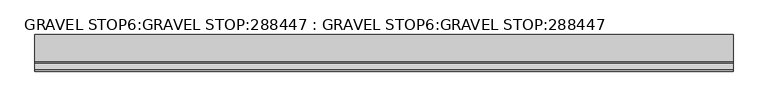
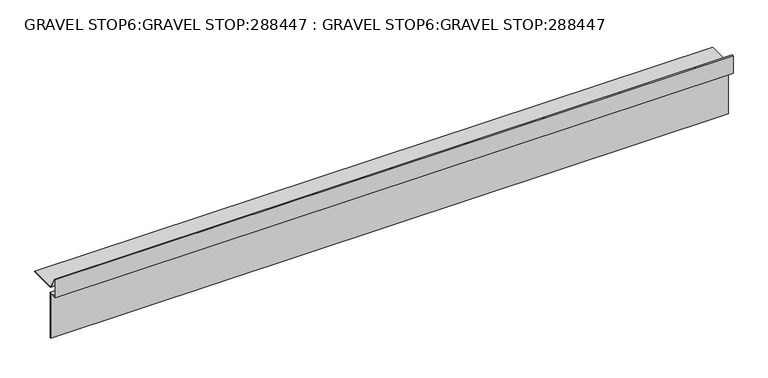
"""IFC4 building model written with IfcOpenShell, lengths in millimetres: proxy geometry, GRAVEL STOP6:GRAVEL STOP:288447 : GRAVEL STOP6:GRAVEL STOP:288447."""

from ifc_helpers import new_model, si_unit, frame, origin, place, context, project, spatial, polyline, outline, extrude, source, transform, mapped, element, save


def gravel_stop6_gravel_stop_288447_gravel_stop6_gravel_stop_baaed02c(model_context):
    return source(origin(), model_context, "Body", "SweptSolid", [
        extrude(outline(polyline([(-5301.703097, 40223.2155287), (-5301.703097, 40278.1940248), (-5298.6711826, 40279.0064238), (-5278.0007291, 40243.204148), (-5274.2484189, 40241.0377507), (-5196.7905122, 40241.0377507), (-5196.7905122, 40239.6266397), (-5274.6265249, 40239.6266397), (-5279.033734, 40242.1711431), (-5299.3518488, 40277.3631503), (-5300.291986, 40277.1112413), (-5300.291986, 40224.6266397), (-5275.9522484, 40224.6266397), (-5275.9522484, 40081.6491197), (-5277.3633594, 40081.6491197), (-5277.3633594, 40223.2155287), (-5301.703097, 40223.2155287)])), frame((17159.7769925, 0.0, 0.0), z_axis=(1.0, 0.0, 0.0), x_axis=(0.0, 1.0, 0.0)), (0.0, 0.0, 1.0), 2000.25),
    ])


if __name__ == "__main__":
    model = new_model("IFC4")
    model_context = context("Model", 3, world=origin())
    ifc_project = project(units=[si_unit("LENGTHUNIT", "METRE", prefix="MILLI")], contexts=[model_context])
    site = spatial("IfcSite", under=ifc_project)
    building = spatial("IfcBuilding", under=site)
    placement = place(None, origin())
    gravel_stop6_gravel_stop_288447_gravel_stop6_gravel_stop_shape = gravel_stop6_gravel_stop_288447_gravel_stop6_gravel_stop_baaed02c(model_context)
    element("IfcBuildingElementProxy", 1, Name="GRAVEL STOP6:GRAVEL STOP:288447 : GRAVEL STOP6:GRAVEL STOP:288447", ObjectType="GRAVEL STOP6:GRAVEL STOP:288447 : GRAVEL STOP6:GRAVEL STOP:288447", at=placement, inside=building, context=model_context, shape_type="MappedRepresentation", body=[
        mapped(gravel_stop6_gravel_stop_288447_gravel_stop6_gravel_stop_shape, transform((0.0, 0.0, 0.0), x_axis=(1.0, 0.0, 0.0), y_axis=(0.0, 1.0, 0.0), z_axis=(0.0, 0.0, 1.0))),
    ])
    save(model, "model.ifc")

# Revit data of these elements
# Type "GRAVEL STOP6:GRAVEL STOP:288447 : GRAVEL STOP6:GRAVEL STOP:288447"
#   NameOverride = "GRAVEL STOP6:GRAVEL STOP:288447"
#   ObjectTypeOverride = "GRAVEL STOP6:GRAVEL STOP"
#   Reference = "GRAVEL STOP"
#   Category = "Generic Models"
#   Tag = "288447"
# Element 1 (IfcBuildingElementProxy, "GRAVEL STOP6:GRAVEL STOP:288447 : GRAVEL STOP6:GRAVEL STOP:288447")
#   Materials on its faces: "GRAVEL STOP REQUIRED WITH GRAVEL SURFACE SYSTEMS"
# Materials
#   "GRAVEL STOP REQUIRED WITH GRAVEL SURFACE SYSTEMS": class "Unassigned", colour RGB 170 170 127, transparency 0, Cost = 0
